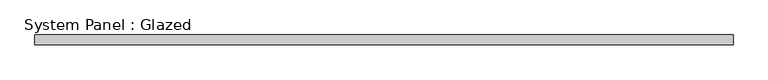
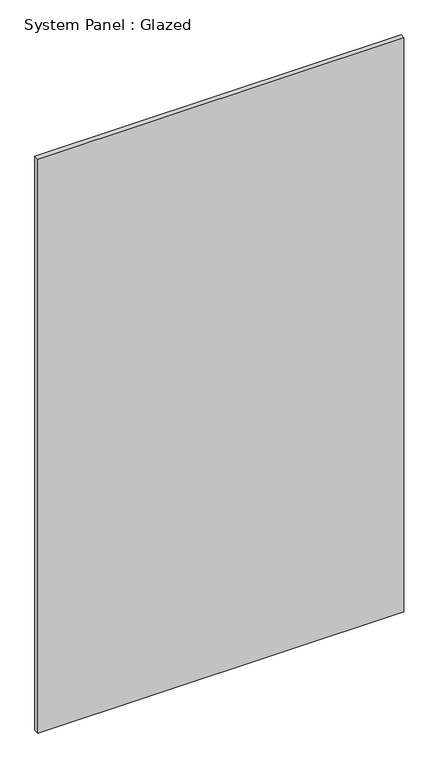
"""IFC4 building model written with IfcOpenShell, lengths in millimetres: plate geometry, System Panel : Glazed."""

from ifc_helpers import new_model, si_unit, origin, origin_with_axes, place, context, project, spatial, polyline, outline, extrude, source, transform, mapped, element, save


def system_panel_glazed_557d3a43(model_context):
    return source(origin(), model_context, "Body", "SweptSolid", [
        extrude(outline(polyline([(904.9999998, 24.5), (-904.9999998, 24.5), (-904.9999998, 49.5), (904.9999998, 49.5), (904.9999998, 24.5)])), origin_with_axes(), (0.0, 0.0, 1.0), 3000.0),
    ])


if __name__ == "__main__":
    model = new_model("IFC4")
    model_context = context("Model", 3, world=origin())
    ifc_project = project(units=[si_unit("LENGTHUNIT", "METRE", prefix="MILLI")], contexts=[model_context])
    site = spatial("IfcSite", under=ifc_project)
    building = spatial("IfcBuilding", under=site)
    placement = place(None, origin())
    system_panel_glazed_shape = system_panel_glazed_557d3a43(model_context)
    element("IfcPlate", 1, ObjectType="System Panel : Glazed", at=placement, inside=building, context=model_context, shape_type="MappedRepresentation", body=[
        mapped(system_panel_glazed_shape, transform((0.0, 0.0, 0.0), x_axis=(1.0, 0.0, 0.0), y_axis=(0.0, 1.0, 0.0), z_axis=(0.0, 0.0, 1.0))),
    ])
    save(model, "model.ifc")

# Revit data of these elements
# Type "System Panel : Glazed"
#   Construction Type Id = "GSP4R"
#   Analytic Construction = "1/8 in Pilkington single glazing"
#   Visual Light Transmittance = 0.9
#   Solar Heat Gain Coefficient = 0.86
#   Heat Transfer Coefficient (U) = 6.7069 W/(m²·K)
#   Define Thermal Properties by = 1
# Element 1 (IfcPlate, "System Panel : Glazed")
#   Materials on its faces: "Glass"
# Materials
#   "Glass": class "Glass", colour RGB 0 128 192, transparency 0.9, Description = "Soda Lime Glass", Cost = 0
